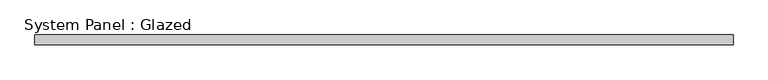
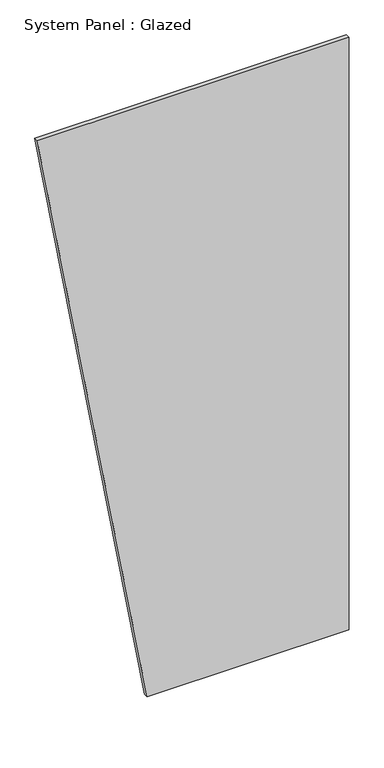
"""IFC4 building model written with IfcOpenShell, lengths in millimetres: plate geometry, System Panel : Glazed."""

import ifcopenshell
import ifcopenshell.guid

model = None  # the IFC model being written
_history = None  # IfcOwnerHistory: only IFC2X3 demands one
_inside = {}  # id of a spatial element -> (the spatial element, [elements in it])
_under = {}  # id of a project, library or spatial element -> (it, [spatial elements below it])
_declared = {}  # id of a project -> (the project, [libraries it declares])
_typed = {}  # id of a type object -> (the type object, [elements of that type])
_made_of = {}  # id of a material, layer set ... -> (it, [elements and type objects made of it])


def new_model(schema):
    """Start an empty IFC model of exactly this schema.

    Asked for "IFC4X3", IfcOpenShell would pick the latest addendum, in which some entities
    have other attributes; the version numbers below select the first issue.
    IFC2X3 requires an IfcOwnerHistory on every rooted entity: one is made here for all.
    """
    global model, _history
    if schema == "IFC4X3":
        model = ifcopenshell.file(schema_version=(4, 3, 0, 0))
    else:
        model = ifcopenshell.file(schema=schema)
    _inside.clear()
    _under.clear()
    _declared.clear()
    _typed.clear()
    _made_of.clear()
    _history = None
    if model.schema == "IFC2X3":
        org = make("IfcOrganization", Name="unknown")
        user = make(
            "IfcPersonAndOrganization",
            ThePerson=make("IfcPerson", FamilyName="unknown"),
            TheOrganization=org,
        )
        app = make(
            "IfcApplication",
            ApplicationDeveloper=org,
            Version="unknown",
            ApplicationFullName="unknown",
            ApplicationIdentifier="unknown",
        )
        _history = make(
            "IfcOwnerHistory",
            OwningUser=user,
            OwningApplication=app,
            ChangeAction="ADDED",
            CreationDate=0,
        )
    return model


def make(cls, **values):
    """One entity of the class cls with the attributes given. An attribute that is None is left unset."""
    return model.create_entity(
        cls, **{name: value for name, value in values.items() if value is not None}
    )


def rooted(cls, **values):
    """An entity with a GlobalId (a new one), such as an element, a storey or a relation."""
    return make(cls, GlobalId=ifcopenshell.guid.new(), OwnerHistory=_history, **values)


def si_unit(unit_type, name, prefix=None):
    """IfcSIUnit, for example si_unit("LENGTHUNIT", "METRE", prefix="MILLI")."""
    return make("IfcSIUnit", UnitType=unit_type, Prefix=prefix, Name=name)


def assignment(units):
    """IfcUnitAssignment: the units of a project."""
    return None if units is None else make("IfcUnitAssignment", Units=units)


def point(xyz):
    """IfcCartesianPoint."""
    return None if xyz is None else make("IfcCartesianPoint", Coordinates=xyz)


def direction(xyz):
    """IfcDirection."""
    return None if xyz is None else make("IfcDirection", DirectionRatios=xyz)


def frame(location, z_axis=None, x_axis=None):
    """IfcAxis2Placement3D, a coordinate frame: its origin and axes. An axis left out is left unset."""
    return make(
        "IfcAxis2Placement3D",
        Location=point(location),
        Axis=direction(z_axis),
        RefDirection=direction(x_axis),
    )


def origin():
    """The frame at (0, 0, 0) with its axes left unset."""
    return frame((0.0, 0.0, 0.0))


def place(relative_to, where):
    """IfcLocalPlacement: puts the frame where relative to a parent placement (None: the world)."""
    return make(
        "IfcLocalPlacement", PlacementRelTo=relative_to, RelativePlacement=where
    )


def context(
    kind, dimensions, precision=None, world=None, true_north=None, identifier=None
):
    """IfcGeometricRepresentationContext, for example the 3D "Model" context."""
    return make(
        "IfcGeometricRepresentationContext",
        ContextIdentifier=identifier,
        ContextType=kind,
        CoordinateSpaceDimension=dimensions,
        Precision=precision,
        WorldCoordinateSystem=world,
        TrueNorth=true_north,
    )


def project(units=None, contexts=None):
    """IfcProject with its units and contexts."""
    return rooted(
        "IfcProject",
        Name="project",
        RepresentationContexts=contexts,
        UnitsInContext=assignment(units),
    )


def spatial(cls, under=None, at=None, **own):
    """A site, building, storey or space (cls), placed at a placement, below another one or the project."""
    s = rooted(cls, ObjectPlacement=at, **own)
    if under is not None:
        _under.setdefault(under.id(), (under, []))[1].append(s)
    return s


def polyline(points):
    """IfcPolyline through the points."""
    return make("IfcPolyline", Points=[point(p) for p in points])


def outline(outer, holes=None, kind="AREA"):
    """IfcArbitraryClosedProfileDef: a profile drawn as a closed curve; with holes, ...WithVoids."""
    if holes is None:
        return make("IfcArbitraryClosedProfileDef", ProfileType=kind, OuterCurve=outer)
    return make(
        "IfcArbitraryProfileDefWithVoids",
        ProfileType=kind,
        OuterCurve=outer,
        InnerCurves=holes,
    )


def extrude(swept, where, along, depth):
    """IfcExtrudedAreaSolid: the profile swept, set in the frame where, extruded along a direction by depth."""
    return make(
        "IfcExtrudedAreaSolid",
        SweptArea=swept,
        Position=where,
        ExtrudedDirection=direction(along),
        Depth=depth,
    )


def shape(context_of_items, identifier, shape_type, items):
    """IfcShapeRepresentation: the items that make up one representation, for example the "Body"."""
    return make(
        "IfcShapeRepresentation",
        ContextOfItems=context_of_items,
        RepresentationIdentifier=identifier,
        RepresentationType=shape_type,
        Items=items,
    )


def source(mapping_origin, context_of_items, identifier, shape_type, items):
    """IfcRepresentationMap: a shape defined once, which mapped items show again and again."""
    return make(
        "IfcRepresentationMap",
        MappingOrigin=mapping_origin,
        MappedRepresentation=shape(context_of_items, identifier, shape_type, items),
    )


def transform(
    local_origin,
    x_axis=None,
    y_axis=None,
    z_axis=None,
    scale=None,
    scale2=None,
    scale3=None,
    uniform=True,
):
    """IfcCartesianTransformationOperator3D, or its non-uniform kind. x_axis, y_axis, z_axis: its Axis1, 2, 3."""
    if uniform:
        return make(
            "IfcCartesianTransformationOperator3D",
            Axis1=direction(x_axis),
            Axis2=direction(y_axis),
            LocalOrigin=point(local_origin),
            Scale=scale,
            Axis3=direction(z_axis),
        )
    return make(
        "IfcCartesianTransformationOperator3DnonUniform",
        Axis1=direction(x_axis),
        Axis2=direction(y_axis),
        LocalOrigin=point(local_origin),
        Scale=scale,
        Axis3=direction(z_axis),
        Scale2=scale2,
        Scale3=scale3,
    )


def mapped(mapping_source, mapping_target):
    """IfcMappedItem: shows the shape of a source again, moved by a transform."""
    return make(
        "IfcMappedItem", MappingSource=mapping_source, MappingTarget=mapping_target
    )


def made_of(thing, what):
    """Note that an element or type object is made of a material, layer set ...; save() writes the relation."""
    if what is not None:
        _made_of.setdefault(what.id(), (what, []))[1].append(thing)
    return thing


def element(
    cls,
    number,
    at=None,
    inside=None,
    cuts=None,
    type_object=None,
    material=None,
    context=None,
    identifier="Body",
    shape_type=None,
    held_by="IfcProductDefinitionShape",
    body=None,
    shapes=None,
    **own,
):
    """One element of the class cls, such as IfcWall. Its Tag is "e" and its number.

    at: its placement. inside: the storey or other place that contains it. cuts: it is an
    opening in that element (IfcRelVoidsElement). A single representation is given by context,
    identifier, shape_type and body (its items); several are given by shapes. held_by: the class
    of the entity that holds the representations. save() writes the other relations.
    """
    e = rooted(cls, Tag="e%d" % number, ObjectPlacement=at, **own)
    if body is not None:
        shapes = [shape(context, identifier, shape_type, body)]
    if shapes is not None:
        e.Representation = make(held_by, Representations=shapes)
    if inside is not None:
        _inside.setdefault(inside.id(), (inside, []))[1].append(e)
    if cuts is not None:
        rooted(
            "IfcRelVoidsElement", RelatingBuildingElement=cuts, RelatedOpeningElement=e
        )
    if type_object is not None:
        _typed.setdefault(type_object.id(), (type_object, []))[1].append(e)
    return made_of(e, material)


def aggregate(whole, parts):
    """IfcRelAggregates: a whole, such as a stair, and the parts it consists of."""
    return rooted("IfcRelAggregates", RelatingObject=whole, RelatedObjects=parts)


def save(model, path):
    """Write the relations noted so far, then the file.

    IfcRelAggregates (storeys below a building ...), IfcRelContainedInSpatialStructure (elements
    in a storey), IfcRelDefinesByType, IfcRelAssociatesMaterial and IfcRelDeclares: one each for
    every whole, place, type object, material and project.
    """
    for whole, parts in _under.values():
        aggregate(whole, parts)
    for where, things in _inside.values():
        rooted(
            "IfcRelContainedInSpatialStructure",
            RelatedElements=things,
            RelatingStructure=where,
        )
    for kind, things in _typed.values():
        rooted("IfcRelDefinesByType", RelatedObjects=things, RelatingType=kind)
    for what, things in _made_of.values():
        rooted("IfcRelAssociatesMaterial", RelatedObjects=things, RelatingMaterial=what)
    for by, libraries in _declared.values():
        rooted("IfcRelDeclares", RelatingContext=by, RelatedDefinitions=libraries)
    model.write(path)


def system_panel_glazed_e7bd2299(model_context):
    return source(origin(), model_context, "Body", "SweptSolid", [
        extrude(outline(polyline([(0.0, -268.2393521), (0.0, 910.7187498), (3657.6, 910.7187498), (3657.6, -910.7187498), (0.0, -268.2393521)])), frame((0.0, -44.45, 0.0), z_axis=(0.0, 1.0, 0.0), x_axis=(0.0, 0.0, 1.0)), (0.0, 0.0, 1.0), 25.4),
    ])


if __name__ == "__main__":
    model = new_model("IFC4")
    model_context = context("Model", 3, world=origin())
    ifc_project = project(units=[si_unit("LENGTHUNIT", "METRE", prefix="MILLI")], contexts=[model_context])
    site = spatial("IfcSite", under=ifc_project)
    building = spatial("IfcBuilding", under=site)
    placement = place(None, origin())
    system_panel_glazed_shape = system_panel_glazed_e7bd2299(model_context)
    element("IfcPlate", 1, ObjectType="System Panel : Glazed", at=placement, inside=building, context=model_context, shape_type="MappedRepresentation", body=[
        mapped(system_panel_glazed_shape, transform((0.0, 0.0, 0.0), x_axis=(1.0, 0.0, 0.0), y_axis=(0.0, 1.0, 0.0), z_axis=(0.0, 0.0, 1.0))),
    ])
    save(model, "model.ifc")

# Revit data of these elements
# Type "System Panel : Glazed"
#   Construction Type Id = "GSP4R"
#   Analytic Construction = "1/8 in Pilkington single glazing"
#   Visual Light Transmittance = 0.9
#   Solar Heat Gain Coefficient = 0.86
#   Heat Transfer Coefficient (U) = 1.18115 BTU/(h·ft²·°F)
#   Define Thermal Properties by = 1
# Element 1 (IfcPlate, "System Panel : Glazed")
#   Materials on its faces: "Glass"
# Materials
#   "Glass": class "Glass", colour RGB 0 128 192, transparency 0.75, Description = "Soda Lime Glass", Cost = 0
